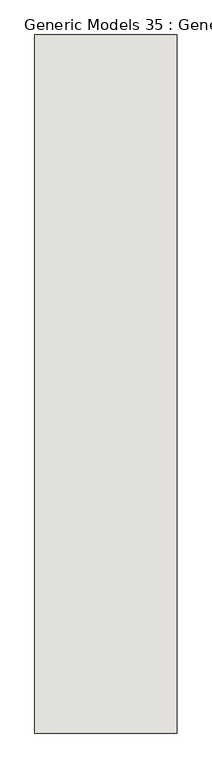
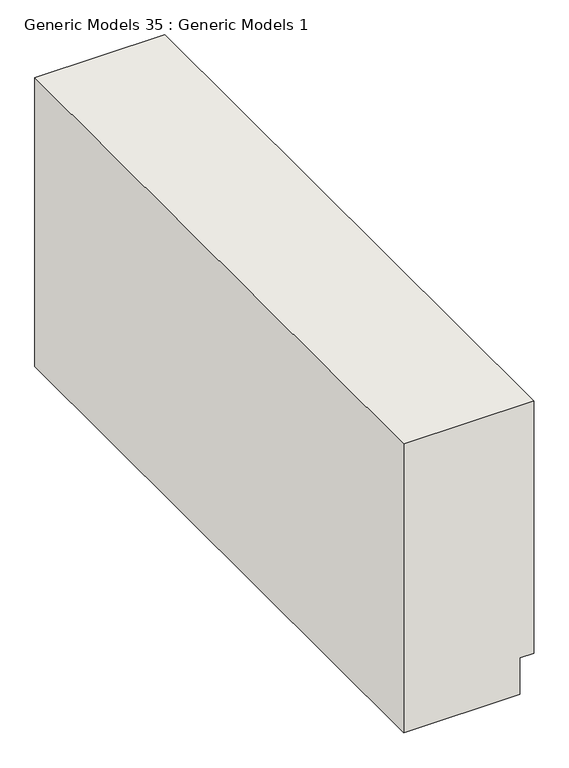
"""IFC4 building model written with IfcOpenShell, lengths in millimetres: wall geometry, Generic Models 35 : Generic Models 1."""

from ifc_helpers import new_model, si_unit, frame, origin, place, context, project, spatial, polyline, outline, extrude, source, transform, mapped, element, save


def generic_models_35_generic_models_1_5be74f3a(model_context):
    return source(origin(), model_context, "Body", "SweptSolid", [
        extrude(outline(polyline([(3035.6238843, 138456.5014063), (3035.6238843, 138208.1931254), (2452.7089811, 138208.1931254), (2452.7089811, 138429.6441211), (2525.961714, 138429.6441211), (2525.961714, 138456.5014063), (3035.6238843, 138456.5014063)])), frame((0.0, 0.0, 0.0), z_axis=(0.0, 1.0, 0.0), x_axis=(0.0, 0.0, 1.0)), (0.0, 0.0, 1.0), 1219.2),
    ])


if __name__ == "__main__":
    model = new_model("IFC4")
    model_context = context("Model", 3, world=origin())
    ifc_project = project(units=[si_unit("LENGTHUNIT", "METRE", prefix="MILLI")], contexts=[model_context])
    site = spatial("IfcSite", under=ifc_project)
    building = spatial("IfcBuilding", under=site)
    placement = place(None, origin())
    generic_models_35_generic_models_1_shape = generic_models_35_generic_models_1_5be74f3a(model_context)
    element("IfcWall", 1, ObjectType="Generic Models 35 : Generic Models 1", at=placement, inside=building, context=model_context, shape_type="MappedRepresentation", body=[
        mapped(generic_models_35_generic_models_1_shape, transform((0.0, 0.0, 0.0), x_axis=(1.0, 0.0, 0.0), y_axis=(0.0, 1.0, 0.0), z_axis=(0.0, 0.0, 1.0))),
    ])
    save(model, "model.ifc")

# Revit data of these elements
# Element 1 (IfcWall, "Generic Models 35 : Generic Models 1")
#   Materials on its faces: "WOOD TRUSS FLOOR ASSEMBLY - FILL CAVITY WITH BATT. INSULATION - (UL - L521 FLOOR ASSEMBLY)"
# Materials
#   "WOOD TRUSS FLOOR ASSEMBLY - FILL CAVITY WITH BATT. INSULATION - (UL - L521 FLOOR ASSEMBLY)": class "Generic", colour RGB 227 188 136, transparency 0, Cost = 0
